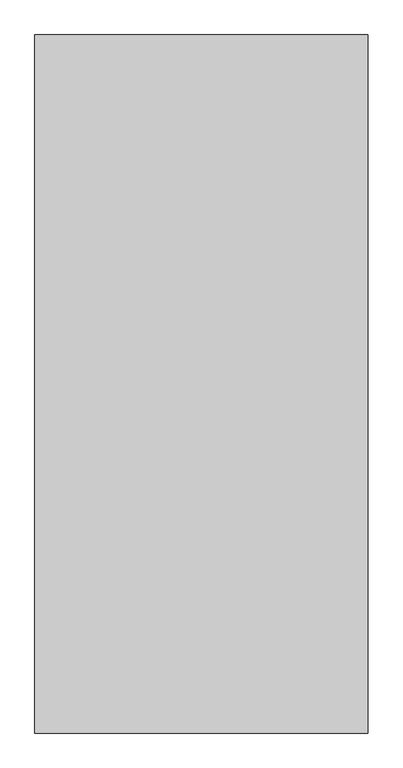
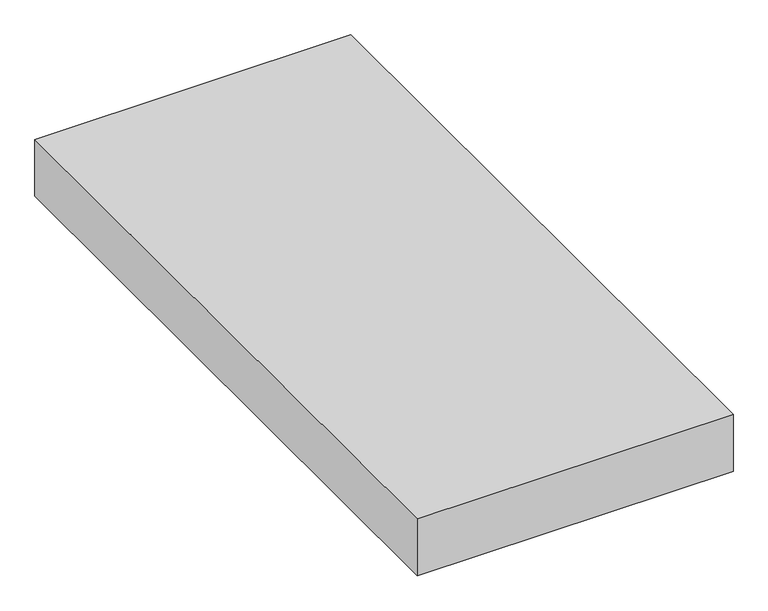
"""IFC4 building model written with IfcOpenShell, lengths in millimetres: proxy geometry, Space Planning Box_hec : Space Planning Box_hec."""

from ifc_helpers import new_model, si_unit, origin, origin_with_axes, place, context, project, spatial, polyline, outline, extrude, source, transform, mapped, element, save


def generic_models_a454a2aa(model_context):
    return source(origin(), model_context, "Body", "SweptSolid", [
        extrude(outline(polyline([(10500.0, 22000.0), (10500.0, -22000.0), (-10500.0, -22000.0), (-10500.0, 22000.0), (10500.0, 22000.0)])), origin_with_axes(), (0.0, 0.0, 1.0), 4000.0),
    ])


if __name__ == "__main__":
    model = new_model("IFC4")
    model_context = context("Model", 3, world=origin())
    ifc_project = project(units=[si_unit("LENGTHUNIT", "METRE", prefix="MILLI")], contexts=[model_context])
    site = spatial("IfcSite", under=ifc_project)
    building = spatial("IfcBuilding", under=site)
    placement = place(None, origin())
    generic_models_shape = generic_models_a454a2aa(model_context)
    element("IfcBuildingElementProxy", 1, Name="Space Planning Box_hec : Space Planning Box_hec", ObjectType="Space Planning Box_hec : Space Planning Box_hec", at=placement, inside=building, context=model_context, shape_type="MappedRepresentation", body=[
        mapped(generic_models_shape, transform((0.0, 0.0, 0.0), x_axis=(1.0, 0.0, 0.0), y_axis=(0.0, 1.0, 0.0), z_axis=(0.0, 0.0, 1.0))),
    ])
    save(model, "model.ifc")

# Revit data of these elements
# Type "Space Planning Box_hec : Space Planning Box_hec"
#   Type Comments = "..."
#   Room Name [instance default] = "?"
#   Interior Finish [instance default] = ""
#   Exterior Finish [instance default] = ""
#   Department [instance default] = ""
#   Assembly Code = "..."
#   Width [instance default] = 1524 mm
#   Program Area [instance default] = 0 m²
#   Length [instance default] = 1524 mm
#   Height [instance default] = 1524 mm
#   Area [instance default] = 2.32258 m²
#   Fill Color [instance default] = Cyan
#   Default Elevation = 0
# Element 1 (IfcBuildingElementProxy, "Space Planning Box_hec : Space Planning Box_hec")
#   Room Name = "Cable Room"
#   Interior Finish = "IF1"
#   Exterior Finish = "EF1"
#   Department = "EL"
#   Width = 21000 mm
#   Program Area = 924 m²
#   Length = 44000 mm
#   Height = 4000 mm
#   Area = 924 m²
#   Fill Color = Blue
#   Materials on its faces: "Blue"
# Materials
#   "Cyan": class "Generic", colour RGB 0 255 255, transparency 0.2, Cost = 0
#   "Blue": class "Generic", colour RGB 0 0 255, transparency 0.2, Cost = 0
